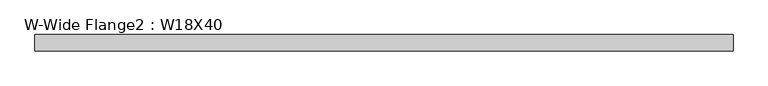
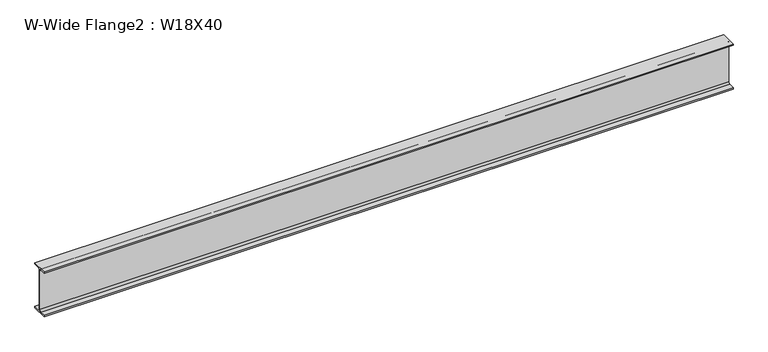
"""IFC4 building model written with IfcOpenShell, lengths in millimetres: beam geometry, W-Wide Flange2 : W18X40."""

import ifcopenshell
import ifcopenshell.guid

model = None  # the IFC model being written
_history = None  # IfcOwnerHistory: only IFC2X3 demands one
_inside = {}  # id of a spatial element -> (the spatial element, [elements in it])
_under = {}  # id of a project, library or spatial element -> (it, [spatial elements below it])
_declared = {}  # id of a project -> (the project, [libraries it declares])
_typed = {}  # id of a type object -> (the type object, [elements of that type])
_made_of = {}  # id of a material, layer set ... -> (it, [elements and type objects made of it])


def new_model(schema):
    """Start an empty IFC model of exactly this schema.

    Asked for "IFC4X3", IfcOpenShell would pick the latest addendum, in which some entities
    have other attributes; the version numbers below select the first issue.
    IFC2X3 requires an IfcOwnerHistory on every rooted entity: one is made here for all.
    """
    global model, _history
    if schema == "IFC4X3":
        model = ifcopenshell.file(schema_version=(4, 3, 0, 0))
    else:
        model = ifcopenshell.file(schema=schema)
    _inside.clear()
    _under.clear()
    _declared.clear()
    _typed.clear()
    _made_of.clear()
    _history = None
    if model.schema == "IFC2X3":
        org = make("IfcOrganization", Name="unknown")
        user = make(
            "IfcPersonAndOrganization",
            ThePerson=make("IfcPerson", FamilyName="unknown"),
            TheOrganization=org,
        )
        app = make(
            "IfcApplication",
            ApplicationDeveloper=org,
            Version="unknown",
            ApplicationFullName="unknown",
            ApplicationIdentifier="unknown",
        )
        _history = make(
            "IfcOwnerHistory",
            OwningUser=user,
            OwningApplication=app,
            ChangeAction="ADDED",
            CreationDate=0,
        )
    return model


def make(cls, **values):
    """One entity of the class cls with the attributes given. An attribute that is None is left unset."""
    return model.create_entity(
        cls, **{name: value for name, value in values.items() if value is not None}
    )


def rooted(cls, **values):
    """An entity with a GlobalId (a new one), such as an element, a storey or a relation."""
    return make(cls, GlobalId=ifcopenshell.guid.new(), OwnerHistory=_history, **values)


def si_unit(unit_type, name, prefix=None):
    """IfcSIUnit, for example si_unit("LENGTHUNIT", "METRE", prefix="MILLI")."""
    return make("IfcSIUnit", UnitType=unit_type, Prefix=prefix, Name=name)


def assignment(units):
    """IfcUnitAssignment: the units of a project."""
    return None if units is None else make("IfcUnitAssignment", Units=units)


def point(xyz):
    """IfcCartesianPoint."""
    return None if xyz is None else make("IfcCartesianPoint", Coordinates=xyz)


def direction(xyz):
    """IfcDirection."""
    return None if xyz is None else make("IfcDirection", DirectionRatios=xyz)


def frame(location, z_axis=None, x_axis=None):
    """IfcAxis2Placement3D, a coordinate frame: its origin and axes. An axis left out is left unset."""
    return make(
        "IfcAxis2Placement3D",
        Location=point(location),
        Axis=direction(z_axis),
        RefDirection=direction(x_axis),
    )


def frame_2d(location, x_axis=None):
    """IfcAxis2Placement2D, a coordinate frame in the plane: its origin and x axis."""
    return make(
        "IfcAxis2Placement2D", Location=point(location), RefDirection=direction(x_axis)
    )


def origin():
    """The frame at (0, 0, 0) with its axes left unset."""
    return frame((0.0, 0.0, 0.0))


def place(relative_to, where):
    """IfcLocalPlacement: puts the frame where relative to a parent placement (None: the world)."""
    return make(
        "IfcLocalPlacement", PlacementRelTo=relative_to, RelativePlacement=where
    )


def context(
    kind, dimensions, precision=None, world=None, true_north=None, identifier=None
):
    """IfcGeometricRepresentationContext, for example the 3D "Model" context."""
    return make(
        "IfcGeometricRepresentationContext",
        ContextIdentifier=identifier,
        ContextType=kind,
        CoordinateSpaceDimension=dimensions,
        Precision=precision,
        WorldCoordinateSystem=world,
        TrueNorth=true_north,
    )


def project(units=None, contexts=None):
    """IfcProject with its units and contexts."""
    return rooted(
        "IfcProject",
        Name="project",
        RepresentationContexts=contexts,
        UnitsInContext=assignment(units),
    )


def spatial(cls, under=None, at=None, **own):
    """A site, building, storey or space (cls), placed at a placement, below another one or the project."""
    s = rooted(cls, ObjectPlacement=at, **own)
    if under is not None:
        _under.setdefault(under.id(), (under, []))[1].append(s)
    return s


def polyline(points):
    """IfcPolyline through the points."""
    return make("IfcPolyline", Points=[point(p) for p in points])


def circle_curve(where, radius):
    """IfcCircle in the frame where."""
    return make("IfcCircle", Position=where, Radius=radius)


def trimmed(basis, trim1, trim2, sense, master):
    """IfcTrimmedCurve: the piece of a basis curve between two trims."""
    return make(
        "IfcTrimmedCurve",
        BasisCurve=basis,
        Trim1=trim1,
        Trim2=trim2,
        SenseAgreement=sense,
        MasterRepresentation=master,
    )


def segment(curve, same_sense, transition):
    """IfcCompositeCurveSegment."""
    return make(
        "IfcCompositeCurveSegment",
        Transition=transition,
        SameSense=same_sense,
        ParentCurve=curve,
    )


def composite_curve(segments, self_intersect=None):
    """IfcCompositeCurve: segments joined end to end."""
    return make("IfcCompositeCurve", Segments=segments, SelfIntersect=self_intersect)


def outline(outer, holes=None, kind="AREA"):
    """IfcArbitraryClosedProfileDef: a profile drawn as a closed curve; with holes, ...WithVoids."""
    if holes is None:
        return make("IfcArbitraryClosedProfileDef", ProfileType=kind, OuterCurve=outer)
    return make(
        "IfcArbitraryProfileDefWithVoids",
        ProfileType=kind,
        OuterCurve=outer,
        InnerCurves=holes,
    )


def extrude(swept, where, along, depth):
    """IfcExtrudedAreaSolid: the profile swept, set in the frame where, extruded along a direction by depth."""
    return make(
        "IfcExtrudedAreaSolid",
        SweptArea=swept,
        Position=where,
        ExtrudedDirection=direction(along),
        Depth=depth,
    )


def shape(context_of_items, identifier, shape_type, items):
    """IfcShapeRepresentation: the items that make up one representation, for example the "Body"."""
    return make(
        "IfcShapeRepresentation",
        ContextOfItems=context_of_items,
        RepresentationIdentifier=identifier,
        RepresentationType=shape_type,
        Items=items,
    )


def source(mapping_origin, context_of_items, identifier, shape_type, items):
    """IfcRepresentationMap: a shape defined once, which mapped items show again and again."""
    return make(
        "IfcRepresentationMap",
        MappingOrigin=mapping_origin,
        MappedRepresentation=shape(context_of_items, identifier, shape_type, items),
    )


def transform(
    local_origin,
    x_axis=None,
    y_axis=None,
    z_axis=None,
    scale=None,
    scale2=None,
    scale3=None,
    uniform=True,
):
    """IfcCartesianTransformationOperator3D, or its non-uniform kind. x_axis, y_axis, z_axis: its Axis1, 2, 3."""
    if uniform:
        return make(
            "IfcCartesianTransformationOperator3D",
            Axis1=direction(x_axis),
            Axis2=direction(y_axis),
            LocalOrigin=point(local_origin),
            Scale=scale,
            Axis3=direction(z_axis),
        )
    return make(
        "IfcCartesianTransformationOperator3DnonUniform",
        Axis1=direction(x_axis),
        Axis2=direction(y_axis),
        LocalOrigin=point(local_origin),
        Scale=scale,
        Axis3=direction(z_axis),
        Scale2=scale2,
        Scale3=scale3,
    )


def mapped(mapping_source, mapping_target):
    """IfcMappedItem: shows the shape of a source again, moved by a transform."""
    return make(
        "IfcMappedItem", MappingSource=mapping_source, MappingTarget=mapping_target
    )


def made_of(thing, what):
    """Note that an element or type object is made of a material, layer set ...; save() writes the relation."""
    if what is not None:
        _made_of.setdefault(what.id(), (what, []))[1].append(thing)
    return thing


def element(
    cls,
    number,
    at=None,
    inside=None,
    cuts=None,
    type_object=None,
    material=None,
    context=None,
    identifier="Body",
    shape_type=None,
    held_by="IfcProductDefinitionShape",
    body=None,
    shapes=None,
    **own,
):
    """One element of the class cls, such as IfcWall. Its Tag is "e" and its number.

    at: its placement. inside: the storey or other place that contains it. cuts: it is an
    opening in that element (IfcRelVoidsElement). A single representation is given by context,
    identifier, shape_type and body (its items); several are given by shapes. held_by: the class
    of the entity that holds the representations. save() writes the other relations.
    """
    e = rooted(cls, Tag="e%d" % number, ObjectPlacement=at, **own)
    if body is not None:
        shapes = [shape(context, identifier, shape_type, body)]
    if shapes is not None:
        e.Representation = make(held_by, Representations=shapes)
    if inside is not None:
        _inside.setdefault(inside.id(), (inside, []))[1].append(e)
    if cuts is not None:
        rooted(
            "IfcRelVoidsElement", RelatingBuildingElement=cuts, RelatedOpeningElement=e
        )
    if type_object is not None:
        _typed.setdefault(type_object.id(), (type_object, []))[1].append(e)
    return made_of(e, material)


def aggregate(whole, parts):
    """IfcRelAggregates: a whole, such as a stair, and the parts it consists of."""
    return rooted("IfcRelAggregates", RelatingObject=whole, RelatedObjects=parts)


def save(model, path):
    """Write the relations noted so far, then the file.

    IfcRelAggregates (storeys below a building ...), IfcRelContainedInSpatialStructure (elements
    in a storey), IfcRelDefinesByType, IfcRelAssociatesMaterial and IfcRelDeclares: one each for
    every whole, place, type object, material and project.
    """
    for whole, parts in _under.values():
        aggregate(whole, parts)
    for where, things in _inside.values():
        rooted(
            "IfcRelContainedInSpatialStructure",
            RelatedElements=things,
            RelatingStructure=where,
        )
    for kind, things in _typed.values():
        rooted("IfcRelDefinesByType", RelatedObjects=things, RelatingType=kind)
    for what, things in _made_of.values():
        rooted("IfcRelAssociatesMaterial", RelatedObjects=things, RelatingMaterial=what)
    for by, libraries in _declared.values():
        rooted("IfcRelDeclares", RelatingContext=by, RelatedDefinitions=libraries)
    model.write(path)


def w_wide_flange2_w18x40_53786035(model_context):
    return source(origin(), model_context, "Body", "SweptSolid", [
        extrude(outline(composite_curve([segment(polyline([(76.454, -213.995), (76.454, -227.33), (-76.454, -227.33), (-76.454, -213.995), (-20.828, -213.995)]), True, "CONTINUOUS"), segment(trimmed(circle_curve(frame_2d((-20.828, -197.1675)), 16.8275), [point((-20.828, -213.995))], [point((-4.0005, -197.1675))], True, "CARTESIAN"), True, "CONTINUOUS"), segment(polyline([(-4.0005, -197.1675), (-4.0005, 197.1675)]), True, "CONTINUOUS"), segment(trimmed(circle_curve(frame_2d((-20.828, 197.1675)), 16.8275), [point((-4.0005, 197.1675))], [point((-20.828, 213.995))], True, "CARTESIAN"), True, "CONTINUOUS"), segment(polyline([(-20.828, 213.995), (-76.454, 213.995), (-76.454, 227.33), (76.454, 227.33), (76.454, 213.995), (20.828, 213.995)]), True, "CONTINUOUS"), segment(trimmed(circle_curve(frame_2d((20.828, 197.1675)), 16.8275), [point((20.828, 213.995))], [point((4.0005, 197.1675))], True, "CARTESIAN"), True, "CONTINUOUS"), segment(polyline([(4.0005, 197.1675), (4.0005, -197.1675)]), True, "CONTINUOUS"), segment(trimmed(circle_curve(frame_2d((20.828, -197.1675)), 16.8275), [point((4.0005, -197.1675))], [point((20.828, -213.995))], True, "CARTESIAN"), True, "CONTINUOUS"), segment(polyline([(20.828, -213.995), (76.454, -213.995)]), True, "CONTINUOUS")], self_intersect=False)), frame((-3289.046, 0.0, 0.0), z_axis=(1.0, 0.0, 0.0), x_axis=(0.0, 1.0, 0.0)), (0.0, 0.0, 1.0), 6578.092),
    ])


if __name__ == "__main__":
    model = new_model("IFC4")
    model_context = context("Model", 3, world=origin())
    ifc_project = project(units=[si_unit("LENGTHUNIT", "METRE", prefix="MILLI")], contexts=[model_context])
    site = spatial("IfcSite", under=ifc_project)
    building = spatial("IfcBuilding", under=site)
    placement = place(None, origin())
    w_wide_flange2_w18x40_shape = w_wide_flange2_w18x40_53786035(model_context)
    element("IfcBeam", 1, ObjectType="W-Wide Flange2 : W18X40", at=placement, inside=building, context=model_context, shape_type="MappedRepresentation", body=[
        mapped(w_wide_flange2_w18x40_shape, transform((0.0, 0.0, 0.0), x_axis=(1.0, 0.0, 0.0), y_axis=(0.0, 1.0, 0.0), z_axis=(0.0, 0.0, 1.0))),
    ])
    save(model, "model.ifc")

# Revit data of these elements
# Type "W-Wide Flange2 : W18X40"
#   Assembly Code = "B10"
#   W = 40
#   Length [instance default] = 5' - 0"
#   bf = 0' - 6.02"
#   d = 1' - 5.9"
#   k = 0' - 1 3/16"
#   k2 = 0' - 0.6625"
#   tf = 0' - 0.525"
#   tw = 0' - 0.315"
#   A = 0.0819444 SF
#   Structural Material [instance default] = Steel ASTM A992
# Element 1 (IfcBeam, "W-Wide Flange2 : W18X40")
#   Materials on its faces: "Steel ASTM A992"
# Materials
#   "Steel ASTM A992": class "Metal", colour RGB 199 199 199, transparency 0, Description = "Structural steel 50ksi", Cost = 0
